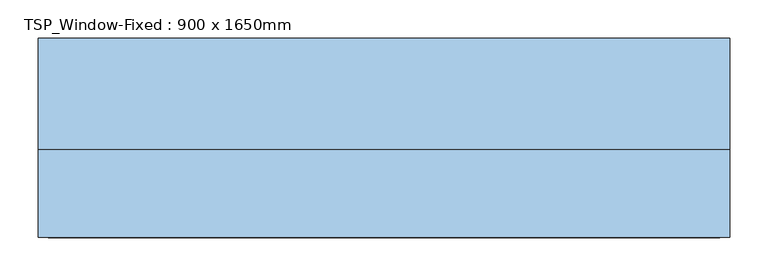
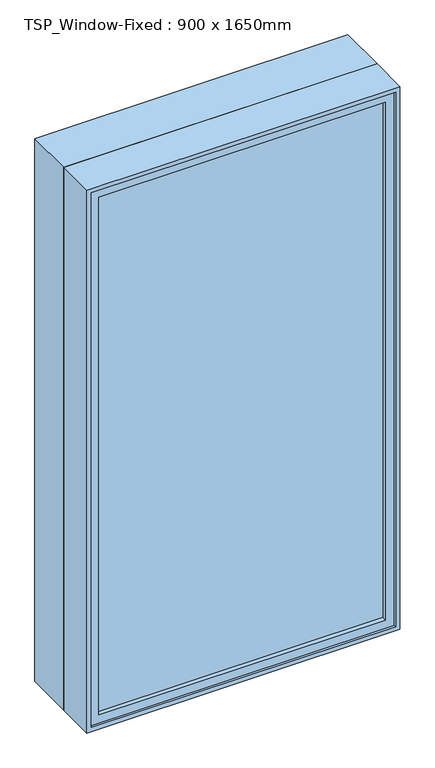
"""IFC4 building model written with IfcOpenShell, lengths in millimetres: window geometry, TSP_Window-Fixed : 900 x 1650mm."""

from ifc_helpers import new_model, si_unit, frame, origin, place, context, project, spatial, polyline, outline, extrude, faceted_brep, source, transform, mapped, element, save


def tsp_window_fixed_900_x_1650mm_280653da(model_context):
    return source(origin(), model_context, "Body", "SolidModel", [
        faceted_brep([(450.0, -24.75, 2550.0), (-450.0, -24.75, 2550.0), (-450.0, -139.05, 2550.0), (450.0, -139.05, 2550.0), (-450.0, -24.75, 900.0), (-450.0, -139.05, 900.0), (450.0, -24.75, 900.0), (450.0, -139.05, 900.0), (418.25, -24.75, 2518.25), (-418.25, -24.75, 2518.25), (-418.25, -24.75, 931.75), (418.25, -24.75, 931.75), (-437.3, -139.05, 2537.3), (437.3, -139.05, 2537.3), (437.3, -139.05, 912.7), (-437.3, -139.05, 912.7), (418.25, -88.25, 2518.25), (-418.25, -88.25, 2518.25), (-437.3, -88.25, 2537.3), (437.3, -88.25, 2537.3), (-418.25, -88.25, 931.75), (-437.3, -88.25, 912.7), (418.25, -88.25, 931.75), (437.3, -88.25, 912.7)], [[[0, 1, 2, 3]], [[1, 4, 5, 2]], [[4, 6, 7, 5]], [[1, 0, 6, 4], [8, 9, 10, 11]], [[6, 0, 3, 7]], [[3, 2, 5, 7], [12, 13, 14, 15]], [[16, 17, 9, 8]], [[13, 12, 18, 19]], [[17, 20, 10, 9]], [[12, 15, 21, 18]], [[20, 22, 11, 10]], [[15, 14, 23, 21]], [[22, 16, 8, 11]], [[19, 18, 21, 23], [17, 16, 22, 20]], [[14, 13, 19, 23]]]),
        extrude(outline(polyline([(2550.0, -450.0), (900.0, -450.0), (900.0, 450.0), (2550.0, 450.0), (2550.0, -450.0)]), holes=[polyline([(2537.3, 437.3), (912.7, 437.3), (912.7, -437.3), (2537.3, -437.3), (2537.3, 437.3)])]), frame((0.0, -24.75, 0.0), z_axis=(0.0, 1.0, 0.0), x_axis=(0.0, 0.0, 1.0)), (0.0, 0.0, 1.0), 144.75),
        extrude(outline(polyline([(912.7, -437.3), (912.7, 437.3), (2537.3, 437.3), (2537.3, -437.3), (912.7, -437.3)]), holes=[polyline([(938.1, 411.9), (938.1, -411.9), (2511.9, -411.9), (2511.9, 411.9), (938.1, 411.9)])]), frame((0.0, -132.7, 0.0), z_axis=(0.0, 1.0, 0.0), x_axis=(0.0, 0.0, 1.0)), (0.0, 0.0, 1.0), 44.45),
        extrude(outline(polyline([(411.9, -120.0), (-411.9, -120.0), (-411.9, -113.65), (411.9, -113.65), (411.9, -120.0)])), frame((0.0, 0.0, 938.1), z_axis=(0.0, 0.0, 1.0), x_axis=(1.0, 0.0, 0.0)), (0.0, 0.0, 1.0), 1573.8),
        extrude(outline(polyline([(-411.9, -100.95), (411.9, -100.95), (411.9, -107.3), (-411.9, -107.3), (-411.9, -100.95)])), frame((0.0, 0.0, 938.1), z_axis=(0.0, 0.0, 1.0), x_axis=(1.0, 0.0, 0.0)), (0.0, 0.0, 1.0), 1573.8),
    ])


if __name__ == "__main__":
    model = new_model("IFC4")
    model_context = context("Model", 3, world=origin())
    ifc_project = project(units=[si_unit("LENGTHUNIT", "METRE", prefix="MILLI")], contexts=[model_context])
    site = spatial("IfcSite", under=ifc_project)
    building = spatial("IfcBuilding", under=site)
    placement = place(None, origin())
    tsp_window_fixed_900_x_1650mm_shape = tsp_window_fixed_900_x_1650mm_280653da(model_context)
    element("IfcWindow", 1, ObjectType="TSP_Window-Fixed : 900 x 1650mm", at=placement, inside=building, context=model_context, shape_type="MappedRepresentation", body=[
        mapped(tsp_window_fixed_900_x_1650mm_shape, transform((0.0, 0.0, 0.0), x_axis=(1.0, 0.0, 0.0), y_axis=(0.0, 1.0, 0.0), z_axis=(0.0, 0.0, 1.0))),
    ])
    save(model, "model.ifc")

# Revit data of these elements
# Type "TSP_Window-Fixed : 900 x 1650mm"
#   Type Mark = "HS 2412 F153"
#   Fire Rating = "0.5h"
#   Assembly Code = "B2020100"
#   Analytic Construction = "Double glazing - domestic"
#   Window Inset [instance default] = 0 mm
#   Wall Thickness [instance default] = 150 mm
#   Visual Light Transmittance = 0.81
#   Thermal Resistance (R) = 0.319569 (m²·K)/W
#   Solar Heat Gain Coefficient = 0.76
#   Rough Width = 915 mm
#   Rough Height = 1665 mm
#   Interior Wall Closure [instance default] = 54.75 mm
#   Height = 1650 mm
#   Heat Transfer Coefficient (U) = 3.12929 W/(m²·K)
#   Frame Extension [instance default] = 6.35 mm
#   Exterior Wall Closure [instance default] = 31.75 mm
#   Extension Jamb [instance default] = 54.75 mm
#   Default Sill Height = 900 mm
#   Width = 900 mm
#   Muntin Visibility = yes
#   Interior Trim Visibility [instance default] = yes
#   Exterior Trim Visibility [instance default] = yes
#   Extension Jamb Visibility [instance default] = yes
#   Interior Trim Material = Wood - Stained
#   Interior Frame Material = Wood - Stained
#   Glass Panel Material = Glass
#   Exterior Trim Material = Clad - White
#   Exterior Frame Material = Clad - White
#   Wall Closure = (empty or 0)
# Element 1 (IfcWindow, "TSP_Window-Fixed : 900 x 1650mm")
#   Wall Thickness = 240 mm
#   Extension Jamb = 144.75 mm
#   Materials on its faces: "Wood - Stained", "Glass", "Clad - White"
# Materials
#   "Wood - Stained": class "Wood", colour RGB 224 178 126, transparency 0, Cost = 0
#   "Glass": class "Glass", colour RGB 0 128 192, transparency 0.9, Description = "Soda Lime Glass", Cost = 0
#   "Clad - White": class "Wood", colour RGB 242 242 238, transparency 0, Cost = 0
